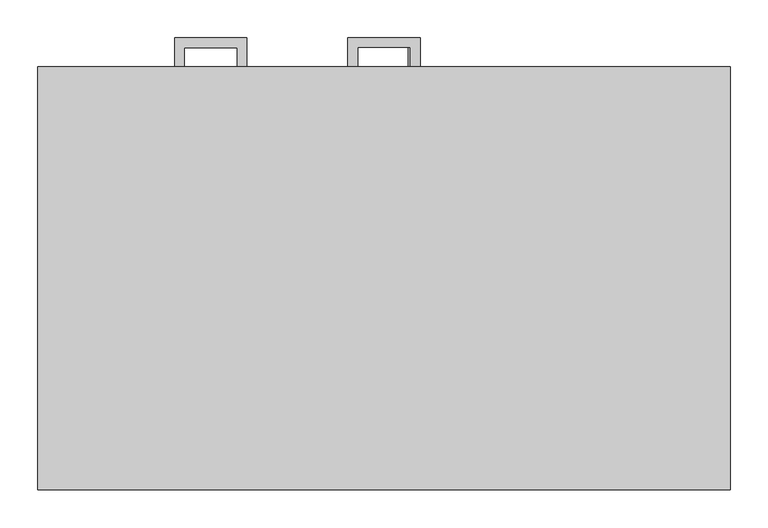
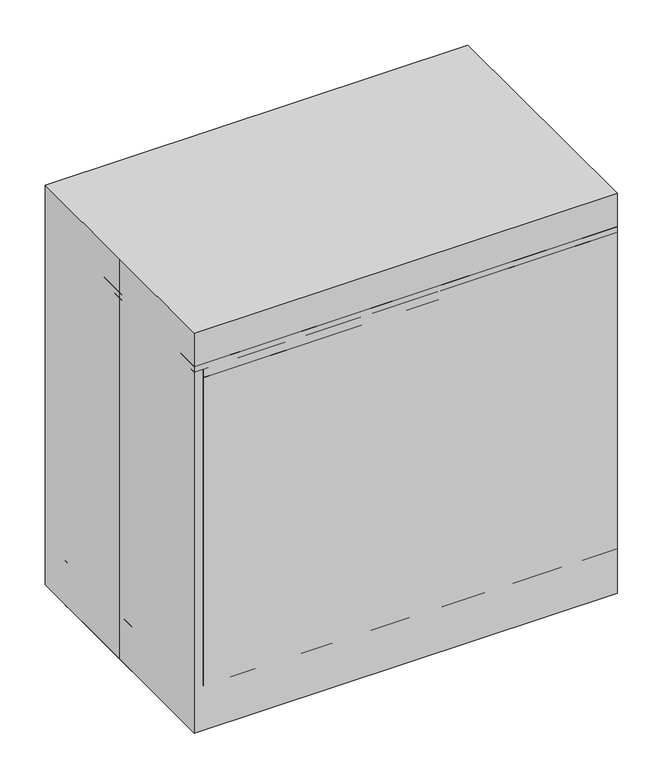
"""IFC4 building model written with IfcOpenShell, lengths in millimetres: proxy geometry, C04L0 - Cabinet, U-C-B, 1 DR, 3 Half DR, 1 Door, 36 W : C04L0 - Cabinet, U-C-B, 1 DR, 3 Half DR, 1 Door, 36 W."""

import ifcopenshell
import ifcopenshell.guid

model = None  # the IFC model being written
_history = None  # IfcOwnerHistory: only IFC2X3 demands one
_inside = {}  # id of a spatial element -> (the spatial element, [elements in it])
_under = {}  # id of a project, library or spatial element -> (it, [spatial elements below it])
_declared = {}  # id of a project -> (the project, [libraries it declares])
_typed = {}  # id of a type object -> (the type object, [elements of that type])
_made_of = {}  # id of a material, layer set ... -> (it, [elements and type objects made of it])


def new_model(schema):
    """Start an empty IFC model of exactly this schema.

    Asked for "IFC4X3", IfcOpenShell would pick the latest addendum, in which some entities
    have other attributes; the version numbers below select the first issue.
    IFC2X3 requires an IfcOwnerHistory on every rooted entity: one is made here for all.
    """
    global model, _history
    if schema == "IFC4X3":
        model = ifcopenshell.file(schema_version=(4, 3, 0, 0))
    else:
        model = ifcopenshell.file(schema=schema)
    _inside.clear()
    _under.clear()
    _declared.clear()
    _typed.clear()
    _made_of.clear()
    _history = None
    if model.schema == "IFC2X3":
        org = make("IfcOrganization", Name="unknown")
        user = make(
            "IfcPersonAndOrganization",
            ThePerson=make("IfcPerson", FamilyName="unknown"),
            TheOrganization=org,
        )
        app = make(
            "IfcApplication",
            ApplicationDeveloper=org,
            Version="unknown",
            ApplicationFullName="unknown",
            ApplicationIdentifier="unknown",
        )
        _history = make(
            "IfcOwnerHistory",
            OwningUser=user,
            OwningApplication=app,
            ChangeAction="ADDED",
            CreationDate=0,
        )
    return model


def make(cls, **values):
    """One entity of the class cls with the attributes given. An attribute that is None is left unset."""
    return model.create_entity(
        cls, **{name: value for name, value in values.items() if value is not None}
    )


def rooted(cls, **values):
    """An entity with a GlobalId (a new one), such as an element, a storey or a relation."""
    return make(cls, GlobalId=ifcopenshell.guid.new(), OwnerHistory=_history, **values)


def si_unit(unit_type, name, prefix=None):
    """IfcSIUnit, for example si_unit("LENGTHUNIT", "METRE", prefix="MILLI")."""
    return make("IfcSIUnit", UnitType=unit_type, Prefix=prefix, Name=name)


def assignment(units):
    """IfcUnitAssignment: the units of a project."""
    return None if units is None else make("IfcUnitAssignment", Units=units)


def point(xyz):
    """IfcCartesianPoint."""
    return None if xyz is None else make("IfcCartesianPoint", Coordinates=xyz)


def direction(xyz):
    """IfcDirection."""
    return None if xyz is None else make("IfcDirection", DirectionRatios=xyz)


def frame(location, z_axis=None, x_axis=None):
    """IfcAxis2Placement3D, a coordinate frame: its origin and axes. An axis left out is left unset."""
    return make(
        "IfcAxis2Placement3D",
        Location=point(location),
        Axis=direction(z_axis),
        RefDirection=direction(x_axis),
    )


def origin():
    """The frame at (0, 0, 0) with its axes left unset."""
    return frame((0.0, 0.0, 0.0))


def origin_with_axes():
    """The frame at (0, 0, 0) with the z axis (0, 0, 1) and the x axis (1, 0, 0) written out."""
    return frame((0.0, 0.0, 0.0), z_axis=(0.0, 0.0, 1.0), x_axis=(1.0, 0.0, 0.0))


def place(relative_to, where):
    """IfcLocalPlacement: puts the frame where relative to a parent placement (None: the world)."""
    return make(
        "IfcLocalPlacement", PlacementRelTo=relative_to, RelativePlacement=where
    )


def context(
    kind, dimensions, precision=None, world=None, true_north=None, identifier=None
):
    """IfcGeometricRepresentationContext, for example the 3D "Model" context."""
    return make(
        "IfcGeometricRepresentationContext",
        ContextIdentifier=identifier,
        ContextType=kind,
        CoordinateSpaceDimension=dimensions,
        Precision=precision,
        WorldCoordinateSystem=world,
        TrueNorth=true_north,
    )


def project(units=None, contexts=None):
    """IfcProject with its units and contexts."""
    return rooted(
        "IfcProject",
        Name="project",
        RepresentationContexts=contexts,
        UnitsInContext=assignment(units),
    )


def spatial(cls, under=None, at=None, **own):
    """A site, building, storey or space (cls), placed at a placement, below another one or the project."""
    s = rooted(cls, ObjectPlacement=at, **own)
    if under is not None:
        _under.setdefault(under.id(), (under, []))[1].append(s)
    return s


def polyline(points):
    """IfcPolyline through the points."""
    return make("IfcPolyline", Points=[point(p) for p in points])


def outline(outer, holes=None, kind="AREA"):
    """IfcArbitraryClosedProfileDef: a profile drawn as a closed curve; with holes, ...WithVoids."""
    if holes is None:
        return make("IfcArbitraryClosedProfileDef", ProfileType=kind, OuterCurve=outer)
    return make(
        "IfcArbitraryProfileDefWithVoids",
        ProfileType=kind,
        OuterCurve=outer,
        InnerCurves=holes,
    )


def extrude(swept, where, along, depth):
    """IfcExtrudedAreaSolid: the profile swept, set in the frame where, extruded along a direction by depth."""
    return make(
        "IfcExtrudedAreaSolid",
        SweptArea=swept,
        Position=where,
        ExtrudedDirection=direction(along),
        Depth=depth,
    )


def shape(context_of_items, identifier, shape_type, items):
    """IfcShapeRepresentation: the items that make up one representation, for example the "Body"."""
    return make(
        "IfcShapeRepresentation",
        ContextOfItems=context_of_items,
        RepresentationIdentifier=identifier,
        RepresentationType=shape_type,
        Items=items,
    )


def source(mapping_origin, context_of_items, identifier, shape_type, items):
    """IfcRepresentationMap: a shape defined once, which mapped items show again and again."""
    return make(
        "IfcRepresentationMap",
        MappingOrigin=mapping_origin,
        MappedRepresentation=shape(context_of_items, identifier, shape_type, items),
    )


def transform(
    local_origin,
    x_axis=None,
    y_axis=None,
    z_axis=None,
    scale=None,
    scale2=None,
    scale3=None,
    uniform=True,
):
    """IfcCartesianTransformationOperator3D, or its non-uniform kind. x_axis, y_axis, z_axis: its Axis1, 2, 3."""
    if uniform:
        return make(
            "IfcCartesianTransformationOperator3D",
            Axis1=direction(x_axis),
            Axis2=direction(y_axis),
            LocalOrigin=point(local_origin),
            Scale=scale,
            Axis3=direction(z_axis),
        )
    return make(
        "IfcCartesianTransformationOperator3DnonUniform",
        Axis1=direction(x_axis),
        Axis2=direction(y_axis),
        LocalOrigin=point(local_origin),
        Scale=scale,
        Axis3=direction(z_axis),
        Scale2=scale2,
        Scale3=scale3,
    )


def mapped(mapping_source, mapping_target):
    """IfcMappedItem: shows the shape of a source again, moved by a transform."""
    return make(
        "IfcMappedItem", MappingSource=mapping_source, MappingTarget=mapping_target
    )


def made_of(thing, what):
    """Note that an element or type object is made of a material, layer set ...; save() writes the relation."""
    if what is not None:
        _made_of.setdefault(what.id(), (what, []))[1].append(thing)
    return thing


def element(
    cls,
    number,
    at=None,
    inside=None,
    cuts=None,
    type_object=None,
    material=None,
    context=None,
    identifier="Body",
    shape_type=None,
    held_by="IfcProductDefinitionShape",
    body=None,
    shapes=None,
    **own,
):
    """One element of the class cls, such as IfcWall. Its Tag is "e" and its number.

    at: its placement. inside: the storey or other place that contains it. cuts: it is an
    opening in that element (IfcRelVoidsElement). A single representation is given by context,
    identifier, shape_type and body (its items); several are given by shapes. held_by: the class
    of the entity that holds the representations. save() writes the other relations.
    """
    e = rooted(cls, Tag="e%d" % number, ObjectPlacement=at, **own)
    if body is not None:
        shapes = [shape(context, identifier, shape_type, body)]
    if shapes is not None:
        e.Representation = make(held_by, Representations=shapes)
    if inside is not None:
        _inside.setdefault(inside.id(), (inside, []))[1].append(e)
    if cuts is not None:
        rooted(
            "IfcRelVoidsElement", RelatingBuildingElement=cuts, RelatedOpeningElement=e
        )
    if type_object is not None:
        _typed.setdefault(type_object.id(), (type_object, []))[1].append(e)
    return made_of(e, material)


def aggregate(whole, parts):
    """IfcRelAggregates: a whole, such as a stair, and the parts it consists of."""
    return rooted("IfcRelAggregates", RelatingObject=whole, RelatedObjects=parts)


def save(model, path):
    """Write the relations noted so far, then the file.

    IfcRelAggregates (storeys below a building ...), IfcRelContainedInSpatialStructure (elements
    in a storey), IfcRelDefinesByType, IfcRelAssociatesMaterial and IfcRelDeclares: one each for
    every whole, place, type object, material and project.
    """
    for whole, parts in _under.values():
        aggregate(whole, parts)
    for where, things in _inside.values():
        rooted(
            "IfcRelContainedInSpatialStructure",
            RelatedElements=things,
            RelatingStructure=where,
        )
    for kind, things in _typed.values():
        rooted("IfcRelDefinesByType", RelatedObjects=things, RelatingType=kind)
    for what, things in _made_of.values():
        rooted("IfcRelAssociatesMaterial", RelatedObjects=things, RelatingMaterial=what)
    for by, libraries in _declared.values():
        rooted("IfcRelDeclares", RelatingContext=by, RelatedDefinitions=libraries)
    model.write(path)


def specialty_equipment_9bda77ac(model_context):
    return source(origin(), model_context, "Body", "SweptSolid", [
        extrude(outline(polyline([(317.5, 614.3543692), (317.5, 519.1043692), (279.4, 519.1043692), (279.4, 531.7884392), (304.8159299, 531.7884392), (304.8159299, 601.6702991), (279.4, 601.6702991), (279.4, 614.3543692), (317.5, 614.3543692)])), frame((31.75, 0.0, 0.0), z_axis=(1.0, 0.0, 0.0), x_axis=(0.0, 1.0, 0.0)), (0.0, 0.0, 1.0), 12.7),
        extrude(outline(polyline([(-180.975, 317.5), (-180.975, 279.4), (-193.6590701, 279.4), (-193.6590701, 304.8159299), (-263.5409299, 304.8159299), (-263.5409299, 279.4), (-276.225, 279.4), (-276.225, 317.5), (-180.975, 317.5)])), frame((0.0, 0.0, 379.4125), z_axis=(0.0, 0.0, 1.0), x_axis=(1.0, 0.0, 0.0)), (0.0, 0.0, 1.0), 12.7),
        extrude(outline(polyline([(-180.975, 317.5), (-180.975, 279.4), (-193.6590701, 279.4), (-193.6590701, 304.8159299), (-263.5409299, 304.8159299), (-263.5409299, 279.4), (-276.225, 279.4), (-276.225, 317.5), (-180.975, 317.5)])), frame((0.0, 0.0, 560.3793692), z_axis=(0.0, 0.0, 1.0), x_axis=(1.0, 0.0, 0.0)), (0.0, 0.0, 1.0), 12.7),
        extrude(outline(polyline([(-180.975, 317.5), (-180.975, 279.4), (-193.6590701, 279.4), (-193.6590701, 304.8159299), (-263.5409299, 304.8159299), (-263.5409299, 279.4), (-276.225, 279.4), (-276.225, 317.5), (-180.975, 317.5)])), frame((0.0, 0.0, 182.5787617), z_axis=(0.0, 0.0, 1.0), x_axis=(1.0, 0.0, 0.0)), (0.0, 0.0, 1.0), 12.7),
        extrude(outline(polyline([(47.625, 317.5), (47.625, 279.4), (34.9409299, 279.4), (34.9409299, 304.8159299), (-34.9409299, 304.8159299), (-34.9409299, 279.4), (-47.625, 279.4), (-47.625, 317.5), (47.625, 317.5)])), frame((0.0, 0.0, 741.3462383), z_axis=(0.0, 0.0, 1.0), x_axis=(1.0, 0.0, 0.0)), (0.0, 0.0, 1.0), 12.7),
        extrude(outline(polyline([(-457.2, -279.4), (-457.2, 0.0), (-457.2, 279.4), (457.2, 279.4), (457.2, -279.4), (-457.2, -279.4)])), origin_with_axes(), (0.0, 0.0, 1.0), 914.4),
        extrude(outline(polyline([(438.15, -279.4), (-438.15, -279.4), (-438.15, 260.35), (438.15, 260.35), (438.15, -279.4)])), frame((0.0, 0.0, 120.7166954), z_axis=(0.0, 0.0, 1.0), x_axis=(1.0, 0.0, 0.0)), (0.0, 0.0, 1.0), 704.7507813),
        extrude(outline(polyline([(-3.175, 279.4), (-3.175, 260.35), (-454.025, 260.35), (-454.025, 279.4), (-3.175, 279.4)])), frame((0.0, 0.0, 285.7418692), z_axis=(0.0, 0.0, 1.0), x_axis=(1.0, 0.0, 0.0)), (0.0, 0.0, 1.0), 174.6168692),
        extrude(outline(polyline([(-3.175, 279.4), (-3.175, 260.35), (-454.025, 260.35), (-454.025, 279.4), (-3.175, 279.4)])), frame((0.0, 0.0, 466.7087383), z_axis=(0.0, 0.0, 1.0), x_axis=(1.0, 0.0, 0.0)), (0.0, 0.0, 1.0), 174.6168692),
        extrude(outline(polyline([(-3.175, 279.4), (-3.175, 260.35), (-454.025, 260.35), (-454.025, 279.4), (-3.175, 279.4)])), frame((0.0, 0.0, 101.6), z_axis=(0.0, 0.0, 1.0), x_axis=(1.0, 0.0, 0.0)), (0.0, 0.0, 1.0), 177.7918692),
        extrude(outline(polyline([(-438.15, -279.4), (-457.2, -279.4), (-457.2, 260.35), (-438.15, 260.35), (-438.15, -279.4)])), frame((0.0, 0.0, 101.6), z_axis=(0.0, 0.0, 1.0), x_axis=(1.0, 0.0, 0.0)), (0.0, 0.0, 1.0), 723.8674767),
        extrude(outline(polyline([(454.025, 279.4), (454.025, 260.35), (-454.025, 260.35), (-454.025, 279.4), (454.025, 279.4)])), frame((0.0, 0.0, 647.6756075), z_axis=(0.0, 0.0, 1.0), x_axis=(1.0, 0.0, 0.0)), (0.0, 0.0, 1.0), 177.7918692),
        extrude(outline(polyline([(454.025, 279.4), (454.025, 260.35), (3.175, 260.35), (3.175, 279.4), (454.025, 279.4)])), frame((0.0, 0.0, 101.6), z_axis=(0.0, 0.0, 1.0), x_axis=(1.0, 0.0, 0.0)), (0.0, 0.0, 1.0), 539.7256075),
        extrude(outline(polyline([(-457.2, 184.15), (-438.15, 184.15), (-438.15, -279.4), (-457.2, -279.4), (-457.2, 184.15)])), origin_with_axes(), (0.0, 0.0, 1.0), 101.6),
        extrude(outline(polyline([(438.15, 184.15), (457.2, 184.15), (457.2, -279.4), (438.15, -279.4), (438.15, 184.15)])), origin_with_axes(), (0.0, 0.0, 1.0), 101.6),
        extrude(outline(polyline([(438.15, 260.35), (457.2, 260.35), (457.2, -279.4), (438.15, -279.4), (438.15, 260.35)])), frame((0.0, 0.0, 101.6), z_axis=(0.0, 0.0, 1.0), x_axis=(1.0, 0.0, 0.0)), (0.0, 0.0, 1.0), 723.8674767),
        extrude(outline(polyline([(-457.2, 260.35), (-438.15, 260.35), (-438.15, -279.4), (-457.2, -279.4), (-457.2, 260.35)])), frame((0.0, 0.0, 101.6), z_axis=(0.0, 0.0, 1.0), x_axis=(1.0, 0.0, 0.0)), (0.0, 0.0, 1.0), 723.8674767),
        extrude(outline(polyline([(457.2, -279.4), (-457.2, -279.4), (-457.2, 260.35), (457.2, 260.35), (457.2, -279.4)])), frame((0.0, 0.0, 825.4674767), z_axis=(0.0, 0.0, 1.0), x_axis=(1.0, 0.0, 0.0)), (0.0, 0.0, 1.0), 12.7325233),
        extrude(outline(polyline([(457.2, 203.2), (457.2, 184.15), (-457.2, 184.15), (-457.2, 203.2), (457.2, 203.2)])), origin_with_axes(), (0.0, 0.0, 1.0), 101.6),
        extrude(outline(polyline([(457.2, -260.35), (457.2, -279.4), (-457.2, -279.4), (-457.2, -260.35), (457.2, -260.35)])), origin_with_axes(), (0.0, 0.0, 1.0), 101.6),
        extrude(outline(polyline([(438.15, -260.35), (-438.15, -260.35), (-438.15, 260.35), (438.15, 260.35), (438.15, -260.35)])), frame((0.0, 0.0, 101.6), z_axis=(0.0, 0.0, 1.0), x_axis=(1.0, 0.0, 0.0)), (0.0, 0.0, 1.0), 19.1166954),
        extrude(outline(polyline([(438.15, -260.35), (438.15, -279.4), (-438.15, -279.4), (-438.15, -260.35), (438.15, -260.35)])), frame((0.0, 0.0, 101.6), z_axis=(0.0, 0.0, 1.0), x_axis=(1.0, 0.0, 0.0)), (0.0, 0.0, 1.0), 704.8174767),
    ])


if __name__ == "__main__":
    model = new_model("IFC4")
    model_context = context("Model", 3, world=origin())
    ifc_project = project(units=[si_unit("LENGTHUNIT", "METRE", prefix="MILLI")], contexts=[model_context])
    site = spatial("IfcSite", under=ifc_project)
    building = spatial("IfcBuilding", under=site)
    placement = place(None, origin())
    specialty_equipment_shape = specialty_equipment_9bda77ac(model_context)
    element("IfcBuildingElementProxy", 1, Name="C04L0 - Cabinet, U-C-B, 1 DR, 3 Half DR, 1 Door, 36 W : C04L0 - Cabinet, U-C-B, 1 DR, 3 Half DR, 1 Door, 36 W", ObjectType="C04L0 - Cabinet, U-C-B, 1 DR, 3 Half DR, 1 Door, 36 W : C04L0 - Cabinet, U-C-B, 1 DR, 3 Half DR, 1 Door, 36 W", at=placement, inside=building, context=model_context, shape_type="MappedRepresentation", body=[
        mapped(specialty_equipment_shape, transform((0.0, 0.0, 0.0), x_axis=(1.0, 0.0, 0.0), y_axis=(0.0, 1.0, 0.0), z_axis=(0.0, 0.0, 1.0))),
    ])
    save(model, "model.ifc")

# Revit data of these elements
# Type "C04L0 - Cabinet, U-C-B, 1 DR, 3 Half DR, 1 Door, 36 W : C04L0 - Cabinet, U-C-B, 1 DR, 3 Half DR, 1 Door, 36 W"
#   Watts2 = "0"
#   Watts1 = "0"
#   Unit_Issue = "EA"
#   UTIL_6_Misc = "-"
#   UTIL_5_NonMedGas = "-"
#   UTIL_4_MiscGas = "-"
#   UTIL_3_MedGas = "-"
#   UTIL_2_Elec = "-"
#   UTIL_1_WaterDrain = "-"
#   Nomenclature = "Cabinet, U/C/B, 1 DR, 3 Half DR, 1 Door, 36\" W"
#   NSN = "6530"
#   Location [instance default] = ""
#   JSN = "C04L0"
#   Fund_Source_VA = "-"
#   Fund_Source_Navy = "-"
#   Fund_Source_Army = "-"
#   Fund_Source_AF = "-"
#   ELEC_Volts2 = "0"
#   ELEC_Volts1 = "0"
#   ELEC_Phase2 = "0"
#   ELEC_Phase1 = "0"
#   ELEC_HertzSwitch = "0"
#   ELEC_HertzDependent = "0"
#   ELEC_Hertz = "0"
#   ELEC_Amps2 = "0"
#   ELEC_Amps1 = "0"
#   DetailDescription = "Standing height under counter base cabinet, 36\" H x 36\" W x 22\" D with a full width drawer above three half width drawers alongside a solid right or left door/cupboard (appropriate door/cupboard configuration to be indicated on equipment elevation drawings). Also referred to as a combination cabinet or a drawer and cupboard cabinet. For general purpose use throughout the facility."
#   CAT_VA = "A"
#   CAT_Navy = "A"
#   CAT_IHS = "-"
#   CAT_Army = "A"
#   CAT_AF = "A"
#   BTUperhour = "0"
#   Weight_IP = 155
#   DIM_Width_IP = 3' - 0"
#   DIM_Height_IP = 3' - 0"
#   DIM_Depth_IP = 1' - 10"
#   Top Panel Material = none
#   Toe Panel Material = none
#   Side Panel Material = none
#   Shelf Panel Material = none
#   Drawer Front Material = none
#   Door Panel Material = none
#   Back Panel Material = none
#   Assembly Code = ""
# Element 1 (IfcBuildingElementProxy, "C04L0 - Cabinet, U-C-B, 1 DR, 3 Half DR, 1 Door, 36 W : C04L0 - Cabinet, U-C-B, 1 DR, 3 Half DR, 1 Door, 36 W")
#   Materials on its faces: "Default metal", "EquipSpace"
# Materials
#   "Default metal": class "Unassigned", colour RGB 204 204 204, transparency 0
#   "EquipSpace": class "Unassigned", colour RGB 221 217 195, transparency 0.5
